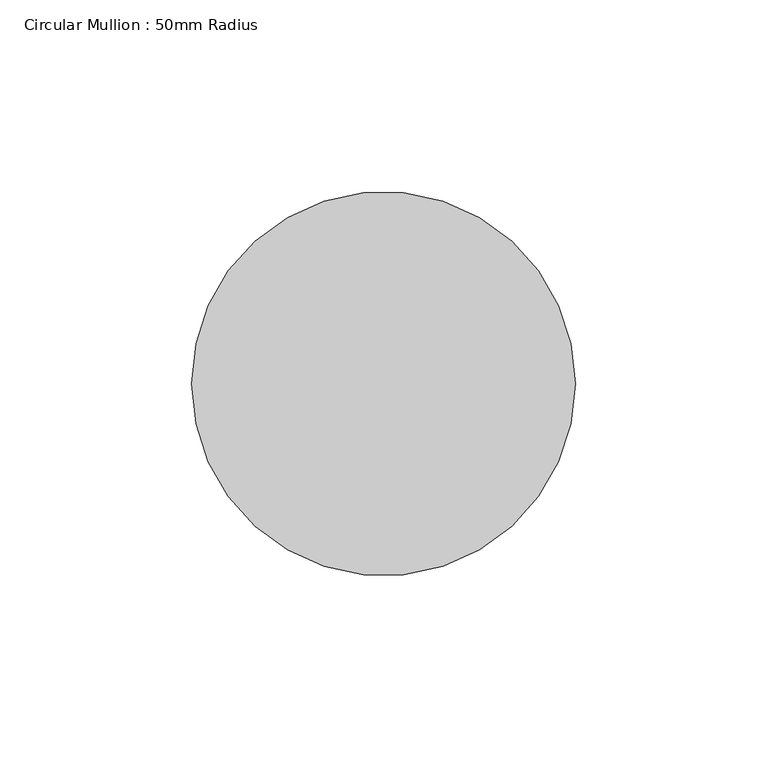
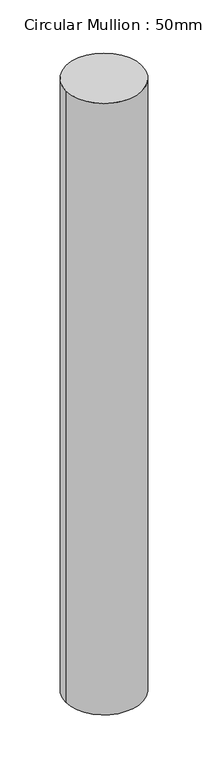
"""IFC4 building model written with IfcOpenShell, lengths in millimetres: member geometry, Circular Mullion : 50mm Radius."""

from ifc_helpers import new_model, si_unit, point, frame, origin, origin_2d, place, context, project, spatial, circle_curve, trimmed, segment, composite_curve, outline, extrude, source, transform, mapped, element, save


def circular_mullion_50mm_radius_983b5c2a(model_context):
    return source(origin(), model_context, "Body", "SweptSolid", [
        extrude(outline(composite_curve([segment(trimmed(circle_curve(origin_2d(), 50.0), [point((50.0, 0.0))], [point((-50.0, 0.0))], False, "CARTESIAN"), True, "CONTINUOUS"), segment(trimmed(circle_curve(origin_2d(), 50.0), [point((-50.0, 0.0))], [point((50.0, 0.0))], False, "CARTESIAN"), True, "CONTINUOUS")], self_intersect=False)), frame((0.0, 0.0, -849.7341422), z_axis=(0.0, 0.0, 1.0), x_axis=(1.0, 0.0, 0.0)), (0.0, 0.0, 1.0), 849.7341422),
    ])


if __name__ == "__main__":
    model = new_model("IFC4")
    model_context = context("Model", 3, world=origin())
    ifc_project = project(units=[si_unit("LENGTHUNIT", "METRE", prefix="MILLI")], contexts=[model_context])
    site = spatial("IfcSite", under=ifc_project)
    building = spatial("IfcBuilding", under=site)
    placement = place(None, origin())
    circular_mullion_50mm_radius_shape = circular_mullion_50mm_radius_983b5c2a(model_context)
    element("IfcMember", 1, ObjectType="Circular Mullion : 50mm Radius", at=placement, inside=building, context=model_context, shape_type="MappedRepresentation", body=[
        mapped(circular_mullion_50mm_radius_shape, transform((0.0, 0.0, 0.0), x_axis=(1.0, 0.0, 0.0), y_axis=(0.0, 1.0, 0.0), z_axis=(0.0, 0.0, 1.0))),
    ])
    save(model, "model.ifc")

# Revit data of these elements
# Type "Circular Mullion : 50mm Radius"
#   built-in parameter 1007350 = 0.164042 (stored number, unit not read)
# Element 1 (IfcMember, "Circular Mullion : 50mm Radius")
#   Materials on its faces: "Aluminium"
# Materials
#   "Aluminium": class "Metal", colour RGB 247 247 247, transparency 0, Description = "Aluminium 6061", Cost = 0
